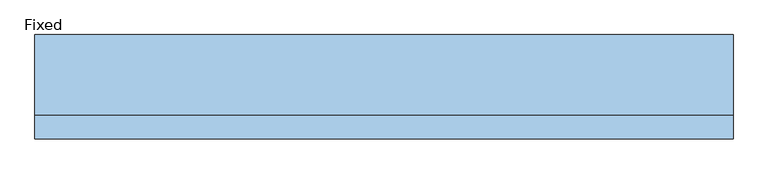
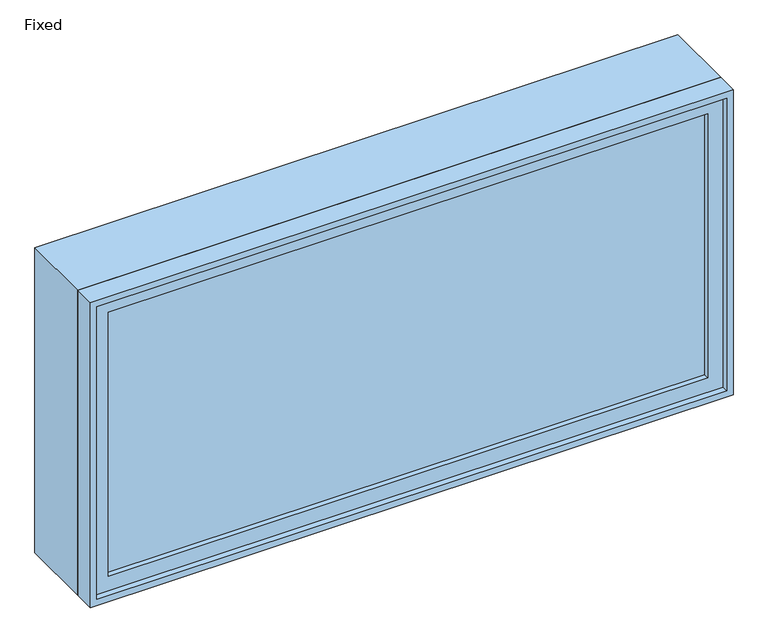
"""IFC4 building model written with IfcOpenShell, lengths in millimetres: window geometry, Fixed."""

from ifc_helpers import new_model, si_unit, frame, origin, place, context, project, spatial, polyline, outline, extrude, source, transform, mapped, element, save


def fixed_06ce57b0(model_context):
    return source(origin(), model_context, "Body", "SweptSolid", [
        extrude(outline(polyline([(835.025, -92.075), (835.025, -104.775), (-911.225, -104.775), (-911.225, -92.075), (835.025, -92.075)])), frame((0.0, 0.0, 1257.3), z_axis=(0.0, 0.0, 1.0), x_axis=(1.0, 0.0, 0.0)), (0.0, 0.0, 1.0), 812.8),
        extrude(outline(polyline([(2114.55, -955.675), (1212.85, -955.675), (1212.85, 879.475), (2114.55, 879.475), (2114.55, -955.675)]), holes=[polyline([(2070.1, -911.225), (2070.1, 835.025), (1257.3, 835.025), (1257.3, -911.225), (2070.1, -911.225)])]), frame((0.0, -120.65, 0.0), z_axis=(0.0, 1.0, 0.0), x_axis=(0.0, 0.0, 1.0)), (0.0, 0.0, 1.0), 44.45),
        extrude(outline(polyline([(2133.6, -974.725), (1193.8, -974.725), (1193.8, 898.525), (2133.6, 898.525), (2133.6, -974.725)]), holes=[polyline([(2101.85, -942.975), (2101.85, 866.775), (1225.55, 866.775), (1225.55, -942.975), (2101.85, -942.975)])]), frame((0.0, -76.2, 0.0), z_axis=(0.0, 1.0, 0.0), x_axis=(0.0, 0.0, 1.0)), (0.0, 0.0, 1.0), 215.9),
        extrude(outline(polyline([(2133.6, 898.525), (2133.6, -974.725), (1193.8, -974.725), (1193.8, 898.525), (2133.6, 898.525)]), holes=[polyline([(2114.55, 879.475), (1212.85, 879.475), (1212.85, -955.675), (2114.55, -955.675), (2114.55, 879.475)])]), frame((0.0, -139.7, 0.0), z_axis=(0.0, 1.0, 0.0), x_axis=(0.0, 0.0, 1.0)), (0.0, 0.0, 1.0), 63.5),
    ])


if __name__ == "__main__":
    model = new_model("IFC4")
    model_context = context("Model", 3, world=origin())
    ifc_project = project(units=[si_unit("LENGTHUNIT", "METRE", prefix="MILLI")], contexts=[model_context])
    site = spatial("IfcSite", under=ifc_project)
    building = spatial("IfcBuilding", under=site)
    placement = place(None, origin())
    fixed_shape = fixed_06ce57b0(model_context)
    element("IfcWindow", 1, ObjectType="Fixed : 6' 1 34\"\" x 3' 1\"", at=placement, inside=building, context=model_context, shape_type="MappedRepresentation", body=[
        mapped(fixed_shape, transform((0.0, 0.0, 0.0), x_axis=(1.0, 0.0, 0.0), y_axis=(0.0, 1.0, 0.0), z_axis=(0.0, 0.0, 1.0))),
    ])
    save(model, "model.ifc")

# Revit data of these elements
# Project information
#   Project Issue Date = "Issue Date"
#   Project Status = "Project Status"
#   Client Name = "Owner"
#   Project Address = "Enter address here"
#   Project Name = "Project Name"
#   Project Number = "Project Number"
# Type "Fixed : 6' 1 34\"\" x 3' 1\""
#   Type Mark = "10"
#   Assembly Code = "B2020100"
#   Height = 3' - 1"
#   Default Sill Height = 3' - 11"
#   Width = 6' - 1 3/4"
#   Window Inset = 0' - 0 3/4"
#   Glass Pane Material = Glass
#   Sash Material = Sash
#   Wall Closure = (empty or 0)
# Element 1 (IfcWindow, "Fixed : 6' 1 34\"\" x 3' 1\"")
#   Materials on its faces: "Sash", "Glass"
# Materials
#   "Glass": class "Glass", colour RGB 218 227 224, transparency 0.85, Description = "Soda Lime Glass", Cost = 0
#   "Sash": class "Wood", colour RGB 136 99 55, transparency 0
